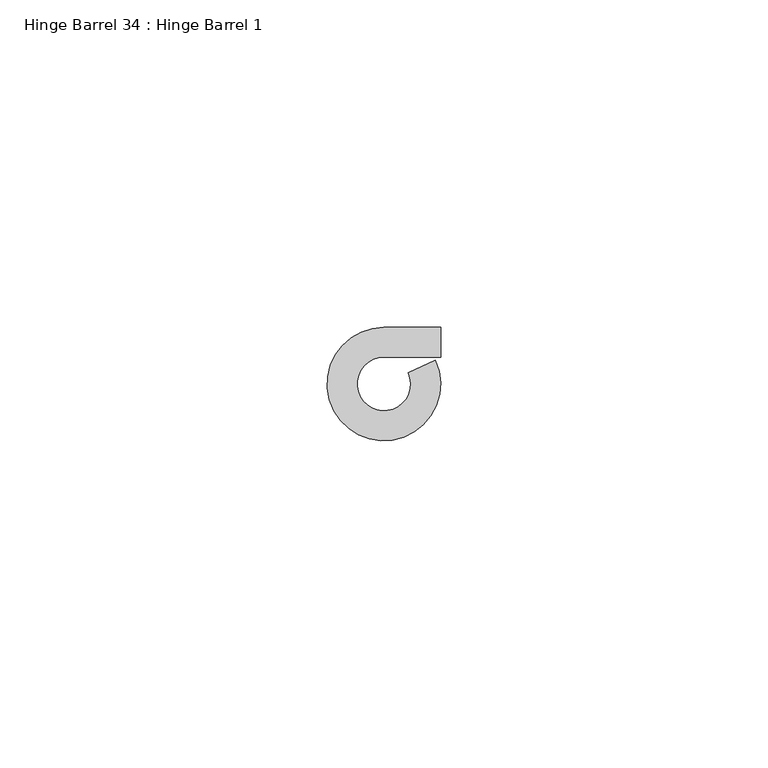
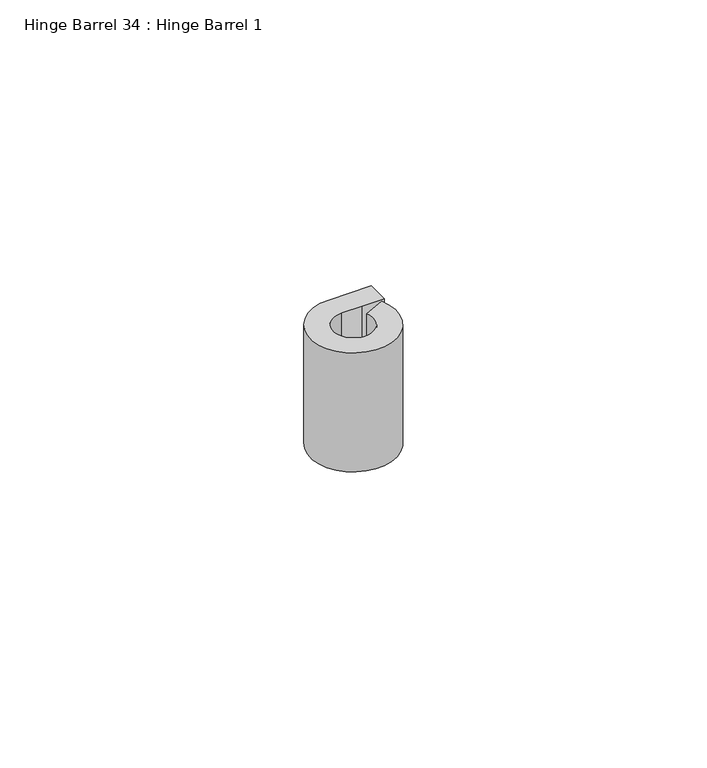
"""IFC4 building model written with IfcOpenShell, lengths in millimetres: proxy geometry, Hinge Barrel 34 : Hinge Barrel 1."""

from ifc_helpers import new_model, si_unit, point, frame, frame_2d, origin, place, context, project, spatial, polyline, circle_curve, trimmed, segment, composite_curve, outline, extrude, source, transform, mapped, element, save


def hinge_barrel_34_hinge_barrel_1_1aaac7a2(model_context):
    return source(origin(), model_context, "Body", "SweptSolid", [
        extrude(outline(composite_curve([segment(polyline([(587323.2214739, -533980.5883841), (587319.1320739, -533980.5883841)]), True, "CONTINUOUS"), segment(trimmed(circle_curve(frame_2d((587319.1320739, -533984.6777841)), 4.0894), [point((587319.1320739, -533980.5883841))], [point((587322.8436736, -533982.9610371))], True, "CARTESIAN"), True, "CONTINUOUS"), segment(polyline([(587322.8436736, -533982.9610371), (587326.986084, -533981.0450249)]), True, "CONTINUOUS"), segment(trimmed(circle_curve(frame_2d((587319.1320739, -533984.6777841)), 8.6534625), [point((587326.986084, -533981.0450249))], [point((587319.1320739, -533976.0243216))], False, "CARTESIAN"), True, "CONTINUOUS"), segment(polyline([(587319.1320739, -533976.0243216), (587327.7934739, -533976.0243216), (587327.7934739, -533980.5883841), (587323.2214739, -533980.5883841)]), True, "CONTINUOUS")], self_intersect=False)), frame((0.0, 0.0, 1225.55), z_axis=(0.0, 0.0, 1.0), x_axis=(1.0, 0.0, 0.0)), (0.0, 0.0, 1.0), 25.4),
    ])


if __name__ == "__main__":
    model = new_model("IFC4")
    model_context = context("Model", 3, world=origin())
    ifc_project = project(units=[si_unit("LENGTHUNIT", "METRE", prefix="MILLI")], contexts=[model_context])
    site = spatial("IfcSite", under=ifc_project)
    building = spatial("IfcBuilding", under=site)
    placement = place(None, origin())
    hinge_barrel_34_hinge_barrel_1_shape = hinge_barrel_34_hinge_barrel_1_1aaac7a2(model_context)
    element("IfcBuildingElementProxy", 1, Name="Hinge Barrel 34 : Hinge Barrel 1", ObjectType="Hinge Barrel 34 : Hinge Barrel 1", at=placement, inside=building, context=model_context, shape_type="MappedRepresentation", body=[
        mapped(hinge_barrel_34_hinge_barrel_1_shape, transform((0.0, 0.0, 0.0), x_axis=(1.0, 0.0, 0.0), y_axis=(0.0, 1.0, 0.0), z_axis=(0.0, 0.0, 1.0))),
    ])
    save(model, "model.ifc")

# Revit data of these elements
# Element 1 (IfcBuildingElementProxy, "Hinge Barrel 34 : Hinge Barrel 1")
#   Materials on its faces: "6\"X6\" WELD-ON STL BUTT HINGE"
# Materials
#   "6\"X6\" WELD-ON STL BUTT HINGE": class "Metal", colour RGB 189 187 185, transparency 0, Description = "Carbon steel", Cost = 0
